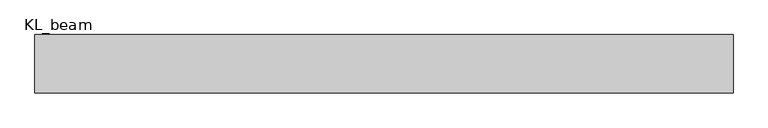
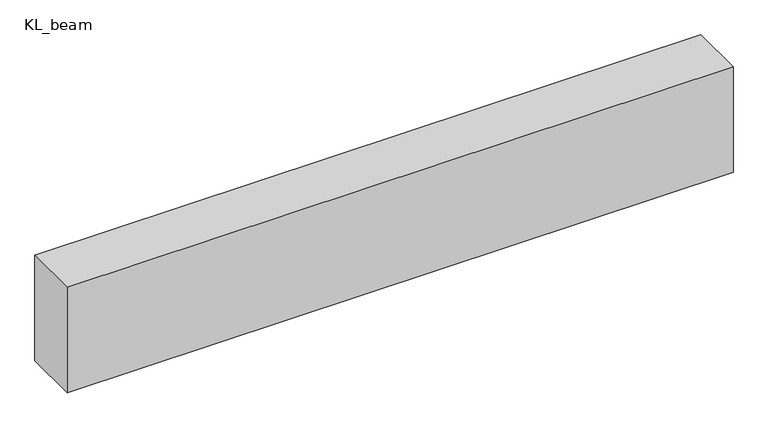
"""IFC4 building model written with IfcOpenShell, lengths in millimetres: beam geometry, 混凝土 - 矩形梁 : KL_beam."""

import ifcopenshell
import ifcopenshell.guid

model = None  # the IFC model being written
_history = None  # IfcOwnerHistory: only IFC2X3 demands one
_inside = {}  # id of a spatial element -> (the spatial element, [elements in it])
_under = {}  # id of a project, library or spatial element -> (it, [spatial elements below it])
_declared = {}  # id of a project -> (the project, [libraries it declares])
_typed = {}  # id of a type object -> (the type object, [elements of that type])
_made_of = {}  # id of a material, layer set ... -> (it, [elements and type objects made of it])


def new_model(schema):
    """Start an empty IFC model of exactly this schema.

    Asked for "IFC4X3", IfcOpenShell would pick the latest addendum, in which some entities
    have other attributes; the version numbers below select the first issue.
    IFC2X3 requires an IfcOwnerHistory on every rooted entity: one is made here for all.
    """
    global model, _history
    if schema == "IFC4X3":
        model = ifcopenshell.file(schema_version=(4, 3, 0, 0))
    else:
        model = ifcopenshell.file(schema=schema)
    _inside.clear()
    _under.clear()
    _declared.clear()
    _typed.clear()
    _made_of.clear()
    _history = None
    if model.schema == "IFC2X3":
        org = make("IfcOrganization", Name="unknown")
        user = make(
            "IfcPersonAndOrganization",
            ThePerson=make("IfcPerson", FamilyName="unknown"),
            TheOrganization=org,
        )
        app = make(
            "IfcApplication",
            ApplicationDeveloper=org,
            Version="unknown",
            ApplicationFullName="unknown",
            ApplicationIdentifier="unknown",
        )
        _history = make(
            "IfcOwnerHistory",
            OwningUser=user,
            OwningApplication=app,
            ChangeAction="ADDED",
            CreationDate=0,
        )
    return model


def make(cls, **values):
    """One entity of the class cls with the attributes given. An attribute that is None is left unset."""
    return model.create_entity(
        cls, **{name: value for name, value in values.items() if value is not None}
    )


def rooted(cls, **values):
    """An entity with a GlobalId (a new one), such as an element, a storey or a relation."""
    return make(cls, GlobalId=ifcopenshell.guid.new(), OwnerHistory=_history, **values)


def si_unit(unit_type, name, prefix=None):
    """IfcSIUnit, for example si_unit("LENGTHUNIT", "METRE", prefix="MILLI")."""
    return make("IfcSIUnit", UnitType=unit_type, Prefix=prefix, Name=name)


def assignment(units):
    """IfcUnitAssignment: the units of a project."""
    return None if units is None else make("IfcUnitAssignment", Units=units)


def point(xyz):
    """IfcCartesianPoint."""
    return None if xyz is None else make("IfcCartesianPoint", Coordinates=xyz)


def direction(xyz):
    """IfcDirection."""
    return None if xyz is None else make("IfcDirection", DirectionRatios=xyz)


def frame(location, z_axis=None, x_axis=None):
    """IfcAxis2Placement3D, a coordinate frame: its origin and axes. An axis left out is left unset."""
    return make(
        "IfcAxis2Placement3D",
        Location=point(location),
        Axis=direction(z_axis),
        RefDirection=direction(x_axis),
    )


def origin():
    """The frame at (0, 0, 0) with its axes left unset."""
    return frame((0.0, 0.0, 0.0))


def place(relative_to, where):
    """IfcLocalPlacement: puts the frame where relative to a parent placement (None: the world)."""
    return make(
        "IfcLocalPlacement", PlacementRelTo=relative_to, RelativePlacement=where
    )


def context(
    kind, dimensions, precision=None, world=None, true_north=None, identifier=None
):
    """IfcGeometricRepresentationContext, for example the 3D "Model" context."""
    return make(
        "IfcGeometricRepresentationContext",
        ContextIdentifier=identifier,
        ContextType=kind,
        CoordinateSpaceDimension=dimensions,
        Precision=precision,
        WorldCoordinateSystem=world,
        TrueNorth=true_north,
    )


def project(units=None, contexts=None):
    """IfcProject with its units and contexts."""
    return rooted(
        "IfcProject",
        Name="project",
        RepresentationContexts=contexts,
        UnitsInContext=assignment(units),
    )


def spatial(cls, under=None, at=None, **own):
    """A site, building, storey or space (cls), placed at a placement, below another one or the project."""
    s = rooted(cls, ObjectPlacement=at, **own)
    if under is not None:
        _under.setdefault(under.id(), (under, []))[1].append(s)
    return s


def polyline(points):
    """IfcPolyline through the points."""
    return make("IfcPolyline", Points=[point(p) for p in points])


def outline(outer, holes=None, kind="AREA"):
    """IfcArbitraryClosedProfileDef: a profile drawn as a closed curve; with holes, ...WithVoids."""
    if holes is None:
        return make("IfcArbitraryClosedProfileDef", ProfileType=kind, OuterCurve=outer)
    return make(
        "IfcArbitraryProfileDefWithVoids",
        ProfileType=kind,
        OuterCurve=outer,
        InnerCurves=holes,
    )


def extrude(swept, where, along, depth):
    """IfcExtrudedAreaSolid: the profile swept, set in the frame where, extruded along a direction by depth."""
    return make(
        "IfcExtrudedAreaSolid",
        SweptArea=swept,
        Position=where,
        ExtrudedDirection=direction(along),
        Depth=depth,
    )


def shape(context_of_items, identifier, shape_type, items):
    """IfcShapeRepresentation: the items that make up one representation, for example the "Body"."""
    return make(
        "IfcShapeRepresentation",
        ContextOfItems=context_of_items,
        RepresentationIdentifier=identifier,
        RepresentationType=shape_type,
        Items=items,
    )


def source(mapping_origin, context_of_items, identifier, shape_type, items):
    """IfcRepresentationMap: a shape defined once, which mapped items show again and again."""
    return make(
        "IfcRepresentationMap",
        MappingOrigin=mapping_origin,
        MappedRepresentation=shape(context_of_items, identifier, shape_type, items),
    )


def transform(
    local_origin,
    x_axis=None,
    y_axis=None,
    z_axis=None,
    scale=None,
    scale2=None,
    scale3=None,
    uniform=True,
):
    """IfcCartesianTransformationOperator3D, or its non-uniform kind. x_axis, y_axis, z_axis: its Axis1, 2, 3."""
    if uniform:
        return make(
            "IfcCartesianTransformationOperator3D",
            Axis1=direction(x_axis),
            Axis2=direction(y_axis),
            LocalOrigin=point(local_origin),
            Scale=scale,
            Axis3=direction(z_axis),
        )
    return make(
        "IfcCartesianTransformationOperator3DnonUniform",
        Axis1=direction(x_axis),
        Axis2=direction(y_axis),
        LocalOrigin=point(local_origin),
        Scale=scale,
        Axis3=direction(z_axis),
        Scale2=scale2,
        Scale3=scale3,
    )


def mapped(mapping_source, mapping_target):
    """IfcMappedItem: shows the shape of a source again, moved by a transform."""
    return make(
        "IfcMappedItem", MappingSource=mapping_source, MappingTarget=mapping_target
    )


def made_of(thing, what):
    """Note that an element or type object is made of a material, layer set ...; save() writes the relation."""
    if what is not None:
        _made_of.setdefault(what.id(), (what, []))[1].append(thing)
    return thing


def element(
    cls,
    number,
    at=None,
    inside=None,
    cuts=None,
    type_object=None,
    material=None,
    context=None,
    identifier="Body",
    shape_type=None,
    held_by="IfcProductDefinitionShape",
    body=None,
    shapes=None,
    **own,
):
    """One element of the class cls, such as IfcWall. Its Tag is "e" and its number.

    at: its placement. inside: the storey or other place that contains it. cuts: it is an
    opening in that element (IfcRelVoidsElement). A single representation is given by context,
    identifier, shape_type and body (its items); several are given by shapes. held_by: the class
    of the entity that holds the representations. save() writes the other relations.
    """
    e = rooted(cls, Tag="e%d" % number, ObjectPlacement=at, **own)
    if body is not None:
        shapes = [shape(context, identifier, shape_type, body)]
    if shapes is not None:
        e.Representation = make(held_by, Representations=shapes)
    if inside is not None:
        _inside.setdefault(inside.id(), (inside, []))[1].append(e)
    if cuts is not None:
        rooted(
            "IfcRelVoidsElement", RelatingBuildingElement=cuts, RelatedOpeningElement=e
        )
    if type_object is not None:
        _typed.setdefault(type_object.id(), (type_object, []))[1].append(e)
    return made_of(e, material)


def aggregate(whole, parts):
    """IfcRelAggregates: a whole, such as a stair, and the parts it consists of."""
    return rooted("IfcRelAggregates", RelatingObject=whole, RelatedObjects=parts)


def save(model, path):
    """Write the relations noted so far, then the file.

    IfcRelAggregates (storeys below a building ...), IfcRelContainedInSpatialStructure (elements
    in a storey), IfcRelDefinesByType, IfcRelAssociatesMaterial and IfcRelDeclares: one each for
    every whole, place, type object, material and project.
    """
    for whole, parts in _under.values():
        aggregate(whole, parts)
    for where, things in _inside.values():
        rooted(
            "IfcRelContainedInSpatialStructure",
            RelatedElements=things,
            RelatingStructure=where,
        )
    for kind, things in _typed.values():
        rooted("IfcRelDefinesByType", RelatedObjects=things, RelatingType=kind)
    for what, things in _made_of.values():
        rooted("IfcRelAssociatesMaterial", RelatedObjects=things, RelatingMaterial=what)
    for by, libraries in _declared.values():
        rooted("IfcRelDeclares", RelatingContext=by, RelatedDefinitions=libraries)
    model.write(path)


def kl_beam_6fd21aec(model_context):
    return source(origin(), model_context, "Body", "SweptSolid", [
        extrude(outline(polyline([(2394.5, 200.0), (2394.5, -200.0), (-2394.5, -200.0), (-2394.5, 200.0), (2394.5, 200.0)])), frame((0.0, 0.0, -400.0), z_axis=(0.0, 0.0, 1.0), x_axis=(1.0, 0.0, 0.0)), (0.0, 0.0, 1.0), 800.0),
    ])


if __name__ == "__main__":
    model = new_model("IFC4")
    model_context = context("Model", 3, world=origin())
    ifc_project = project(units=[si_unit("LENGTHUNIT", "METRE", prefix="MILLI")], contexts=[model_context])
    site = spatial("IfcSite", under=ifc_project)
    building = spatial("IfcBuilding", under=site)
    placement = place(None, origin())
    kl_beam_shape = kl_beam_6fd21aec(model_context)
    element("IfcBeam", 1, ObjectType="混凝土 - 矩形梁 : KL_beam", at=placement, inside=building, context=model_context, shape_type="MappedRepresentation", body=[
        mapped(kl_beam_shape, transform((0.0, 0.0, 0.0), x_axis=(1.0, 0.0, 0.0), y_axis=(0.0, 1.0, 0.0), z_axis=(0.0, 0.0, 1.0))),
    ])
    save(model, "model.ifc")

# Revit data of these elements
# Type "混凝土 - 矩形梁 : KL_beam"
#   Length [instance default] = 1524 mm
#   b = 400 mm
#   h = 800 mm
#   Structural Material [instance default] = 混凝土 - 现场浇注混凝土
#   Assembly Code = ""
# Element 1 (IfcBeam, "混凝土 - 矩形梁 : KL_beam")
#   Structural Material = none
# Materials
#   "混凝土 - 现场浇注混凝土": class "混凝土", colour RGB 192 192 192, transparency 0
